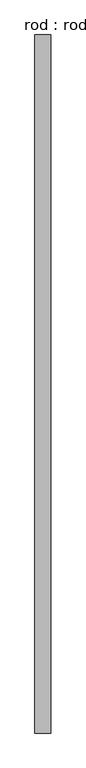
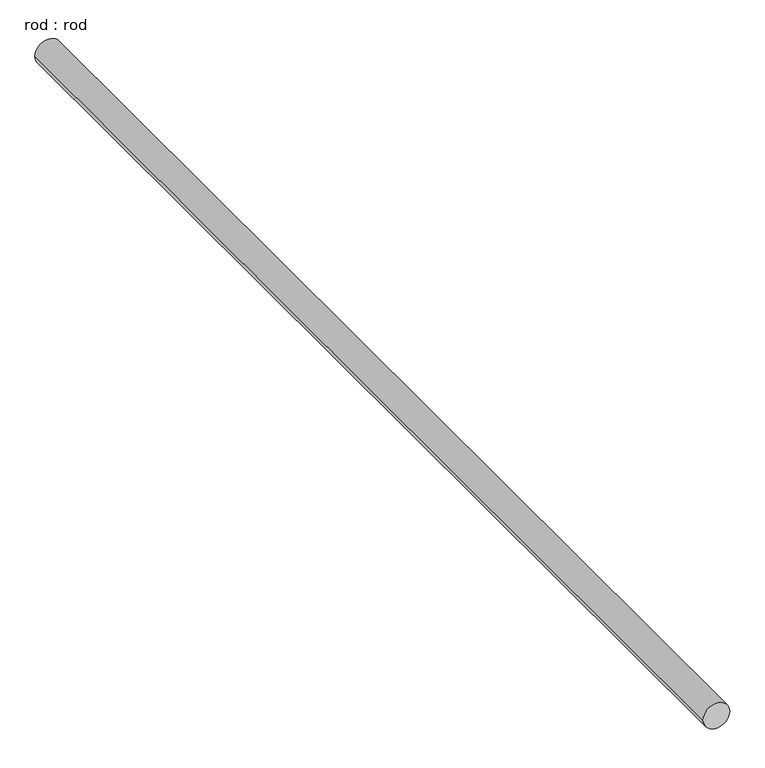
"""IFC4 building model written with IfcOpenShell, lengths in millimetres: proxy geometry, rod : rod."""

from ifc_helpers import new_model, si_unit, point, frame, frame_2d, origin, place, context, project, spatial, circle_curve, trimmed, segment, composite_curve, outline, extrude, source, transform, mapped, element, save


def rod_rod_3872868b(model_context):
    return source(origin(), model_context, "Body", "SweptSolid", [
        extrude(outline(composite_curve([segment(trimmed(circle_curve(frame_2d((0.0108462, 0.0)), 200.0), [point((0.0108462, 200.0))], [point((0.0108462, -200.0))], False, "CARTESIAN"), True, "CONTINUOUS"), segment(trimmed(circle_curve(frame_2d((0.0108462, 0.0)), 200.0), [point((0.0108462, -200.0))], [point((0.0108462, 200.0))], False, "CARTESIAN"), True, "CONTINUOUS")], self_intersect=False)), frame((0.0, -4615.7850638, 0.0), z_axis=(0.0, 1.0, 0.0), x_axis=(0.0, 0.0, 1.0)), (0.0, 0.0, 1.0), 17417.0273582),
    ])


if __name__ == "__main__":
    model = new_model("IFC4")
    model_context = context("Model", 3, world=origin())
    ifc_project = project(units=[si_unit("LENGTHUNIT", "METRE", prefix="MILLI")], contexts=[model_context])
    site = spatial("IfcSite", under=ifc_project)
    building = spatial("IfcBuilding", under=site)
    placement = place(None, origin())
    rod_rod_shape = rod_rod_3872868b(model_context)
    element("IfcBuildingElementProxy", 1, Name="rod : rod", ObjectType="rod : rod", at=placement, inside=building, context=model_context, shape_type="MappedRepresentation", body=[
        mapped(rod_rod_shape, transform((0.0, 0.0, 0.0), x_axis=(1.0, 0.0, 0.0), y_axis=(0.0, 1.0, 0.0), z_axis=(0.0, 0.0, 1.0))),
    ])
    save(model, "model.ifc")

# Revit data of these elements
# Type "rod : rod"
#   Default Elevation = 0
